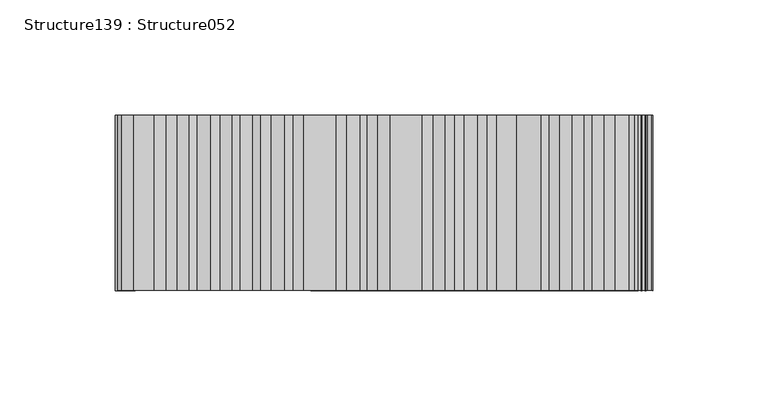
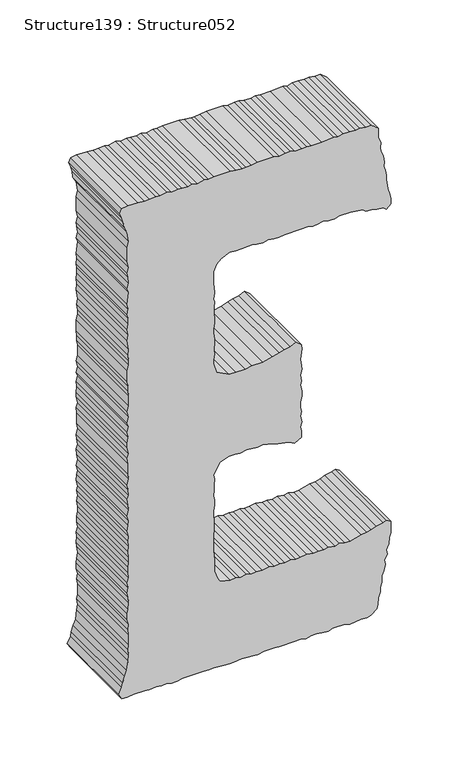
"""IFC4 building model written with IfcOpenShell, lengths in millimetres: proxy geometry, Structure139 : Structure052."""

from ifc_helpers import new_model, si_unit, frame, origin, place, context, project, spatial, polyline, outline, extrude, source, transform, mapped, element, save


def structure139_structure052_afdb430f(model_context):
    return source(origin(), model_context, "Body", "SweptSolid", [
        extrude(outline(polyline([(3552.242032, -42297.2179571), (3556.3417965, -42291.9580636), (3559.8671125, -42291.3563369), (3565.7094775, -42290.7770747), (3570.4109687, -42289.0152189), (3574.5107332, -42289.0152189), (3578.6104977, -42287.83423), (3584.4689087, -42287.83423), (3588.5702778, -42286.0964433), (3593.8285667, -42284.9154544), (3598.5284533, -42285.5171811), (3602.6298224, -42283.1552033), (3606.7295868, -42283.75693), (3611.4134274, -42281.9742144), (3617.2718384, -42281.3933476), (3620.7971545, -42280.2123587), (3625.472972, -42280.2123587), (3631.3410106, -42280.2123587), (3633.6821286, -42283.75693), (3632.5155811, -42286.6532411), (3631.3410106, -42292.5373258), (3629.5984101, -42296.6370903), (3628.4158166, -42300.7384594), (3627.8397636, -42305.4190907), (3625.472972, -42314.8012132), (3625.472972, -42319.4818445), (3626.6571701, -42324.1608712), (3625.472972, -42327.6829781), (3626.6571701, -42333.5429937), (3625.472972, -42337.6668272), (3626.0554434, -42342.3249941), (3625.472972, -42346.4247586), (3626.6571701, -42352.3088433), (3626.0554434, -42357.5687368), (3625.472972, -42361.6685013), (3626.6571701, -42365.7698704), (3625.472972, -42371.0506238), (3626.0554434, -42375.1519929), (3625.472972, -42379.8326242), (3626.6571701, -42384.5116509), (3625.472972, -42390.3957356), (3626.0554434, -42395.6556291), (3625.472972, -42400.3346558), (3626.6571701, -42403.8567627), (3625.472972, -42409.7183829), (3626.6571701, -42413.2388852), (3626.0554434, -42417.9195165), (3628.4158166, -42426.7223767), (3631.915459, -42429.0394256), (3638.9580681, -42431.4030081), (3648.9258713, -42431.4030081), (3654.1841602, -42431.9822703), (3657.7014533, -42432.5615325), (3671.7690209, -42432.5615325), (3677.0449605, -42431.9822703), (3685.8285655, -42431.9822703), (3689.3458585, -42432.5615325), (3694.029699, -42432.5615325), (3699.3136616, -42431.4030081), (3704.0135482, -42431.4030081), (3708.087639, -42432.5615325), (3712.2146818, -42431.9822703), (3716.8985223, -42431.9822703), (3722.7312597, -42431.4030081), (3726.2742264, -42432.5615325), (3733.8736333, -42428.4826279), (3736.2163558, -42426.7223767), (3739.1592005, -42419.1005054), (3739.1592005, -42413.7956829), (3738.5574738, -42409.7183829), (3739.7416719, -42403.8567627), (3739.1592005, -42400.3346558), (3738.5574738, -42394.4746402), (3739.1592005, -42390.3957356), (3737.400554, -42381.5928753), (3735.6146291, -42376.8897795), (3734.47536, -42371.0506238), (3733.2991849, -42366.9508593), (3730.9323932, -42362.8270257), (3734.47536, -42356.9894746), (3739.7416719, -42356.9894746), (3744.4158848, -42357.5687368), (3748.5429276, -42356.3877479), (3753.8012165, -42357.5687368), (3757.8753073, -42356.9894746), (3762.0023501, -42357.5687368), (3766.684586, -42357.5687368), (3771.3860772, -42356.3877479), (3776.6427615, -42356.3877479), (3781.9299333, -42357.5687368), (3785.4456218, -42356.9894746), (3791.3056374, -42357.5687368), (3795.960595, -42356.3877479), (3799.5051664, -42356.9894746), (3805.3459267, -42357.5687368), (3814.7296538, -42356.3877479), (3818.2309008, -42356.9894746), (3822.348316, -42361.6685013), (3820.015221, -42366.3715971), (3818.8310229, -42371.6314906), (3817.6741031, -42375.7312551), (3815.9154565, -42381.5928753), (3814.148787, -42389.7940089), (3814.148787, -42399.1536669), (3812.9726119, -42405.0377516), (3812.9726119, -42413.2388852), (3813.5743386, -42419.1005054), (3818.8310229, -42429.6186879), (3827.6162325, -42432.5615325), (3831.1575946, -42432.5615325), (3835.8334121, -42431.4030081), (3840.5172527, -42431.9822703), (3845.8012153, -42431.4030081), (3849.8753061, -42431.4030081), (3855.1769193, -42432.5615325), (3859.2606378, -42432.5615325), (3863.9332461, -42431.4030081), (3868.0618934, -42431.4030081), (3873.3185778, -42431.9822703), (3878.5784713, -42431.9822703), (3883.2863809, -42431.4030081), (3886.2051565, -42432.5615325), (3891.5067697, -42431.4030081), (3896.763454, -42431.9822703), (3900.2887701, -42432.5615325), (3910.8310217, -42432.5615325), (3916.6653636, -42429.6186879), (3920.7908018, -42426.1206501), (3923.7079727, -42418.4987787), (3923.1319197, -42413.2388852), (3923.7079727, -42408.537394), (3923.7079727, -42399.1536669), (3923.1319197, -42395.6556291), (3922.5494483, -42389.7940089), (3923.7079727, -42385.6926398), (3922.5494483, -42380.4118864), (3922.5494483, -42376.3105173), (3923.1319197, -42371.6314906), (3923.1319197, -42357.5687368), (3923.7079727, -42351.7071166), (3922.5494483, -42347.0040208), (3922.5494483, -42342.9267208), (3923.7079727, -42338.2460895), (3922.5494483, -42333.5429937), (3922.5494483, -42328.2847047), (3923.7079727, -42324.1608712), (3923.7079727, -42314.8012132), (3922.5494483, -42304.2381018), (3920.2067257, -42301.3177216), (3919.6066036, -42296.6370903), (3918.4480792, -42291.9580636), (3917.8479571, -42286.6532411), (3915.5068392, -42283.75693), (3919.6066036, -42280.2123587), (3924.2888396, -42280.2123587), (3928.4158823, -42280.8140853), (3933.6741713, -42282.5759411), (3937.1930689, -42283.1552033), (3942.4770315, -42283.75693), (3946.5511223, -42283.75693), (3951.2606365, -42284.9154544), (3955.360401, -42286.0964433), (3959.4617701, -42285.5171811), (3965.3201811, -42286.6532411), (3969.994394, -42288.4359567), (3973.5197101, -42289.0152189), (3977.6194746, -42288.4359567), (3983.4794902, -42290.7770747), (3988.1633307, -42290.7770747), (3991.6806238, -42290.7770747), (3996.390138, -42296.6370903), (3996.390138, -42301.3177216), (3996.9645864, -42306.6000796), (3996.390138, -42310.0981174), (3996.9645864, -42315.3804754), (3996.9645864, -42320.6628334), (3995.7803883, -42325.3418601), (3996.9645864, -42328.863967), (3995.7803883, -42339.4046139), (3995.7803883, -42348.1850097), (3996.390138, -42352.3088433), (3995.7803883, -42356.3877479), (3995.7803883, -42362.2477635), (3996.9645864, -42366.3715971), (3996.9645864, -42370.4488971), (3995.7803883, -42375.7312551), (3996.9645864, -42380.4118864), (3996.9645864, -42394.4746402), (3996.390138, -42399.7553936), (3995.7803883, -42404.4584894), (3995.7803883, -42407.3548005), (3996.390138, -42413.2388852), (3996.9645864, -42417.9195165), (3996.9645864, -42431.9822703), (3996.390138, -42436.661297), (3996.9645864, -42440.1834039), (3995.7803883, -42446.0450241), (3996.9645864, -42450.7465153), (3995.7803883, -42454.2461577), (3996.390138, -42459.5044466), (3996.390138, -42463.0265535), (3995.7803883, -42468.3089115), (3996.9645864, -42472.4086759), (3995.7803883, -42478.2702962), (3996.390138, -42481.768334), (3995.7803883, -42487.0731564), (3995.7803883, -42491.7537877), (3996.390138, -42497.0120767), (3996.390138, -42505.7940771), (3995.7803883, -42511.0972949), (3991.6806238, -42512.8366862), (3987.5792547, -42511.0972949), (3982.8793681, -42509.916306), (3977.6194746, -42509.3370438), (3972.3627903, -42506.3958038), (3964.1343784, -42505.2148149), (3958.8776941, -42506.3958038), (3945.9766739, -42506.3958038), (3940.718385, -42505.2148149), (3935.4328178, -42506.3958038), (3931.9058971, -42505.7940771), (3926.0490907, -42505.2148149), (3921.3748778, -42506.3958038), (3917.8479571, -42505.2148149), (3907.3313793, -42506.3958038), (3902.6314927, -42505.7940771), (3897.9476522, -42506.3958038), (3894.4030808, -42505.7940771), (3889.7208449, -42505.7940771), (3884.4609514, -42506.3958038), (3879.7610648, -42505.7940771), (3874.5043805, -42506.3958038), (3866.3032469, -42505.2148149), (3861.0192843, -42505.7940771), (3855.7353217, -42505.2148149), (3852.2340747, -42505.2148149), (3846.9757858, -42506.3958038), (3836.9919366, -42506.3958038), (3832.8921721, -42505.7940771), (3828.2163546, -42505.7940771), (3824.1149855, -42505.2148149), (3814.7296538, -42505.2148149), (3810.0474179, -42506.3958038), (3804.7730829, -42505.2148149), (3799.5051664, -42506.3958038), (3795.960595, -42505.2148149), (3791.3056374, -42506.3958038), (3786.6298199, -42505.7940771), (3781.3282066, -42506.3958038), (3777.2444882, -42506.3958038), (3771.3860772, -42505.2148149), (3767.8607611, -42506.3958038), (3762.5848215, -42505.7940771), (3753.2171405, -42505.7940771), (3748.5429276, -42505.2148149), (3743.2332913, -42506.3958038), (3739.1592005, -42505.7940771), (3733.8736333, -42505.2148149), (3730.3563402, -42506.3958038), (3725.0996559, -42505.7940771), (3720.4158154, -42505.2148149), (3715.1302482, -42506.3958038), (3710.4560353, -42505.2148149), (3706.9130685, -42505.7940771), (3701.6547796, -42506.3958038), (3696.3884676, -42505.2148149), (3692.2710525, -42505.7940771), (3687.587212, -42505.2148149), (3682.8857208, -42505.7940771), (3677.6274319, -42505.2148149), (3672.9435914, -42505.2148149), (3668.8261762, -42505.7940771), (3663.5598643, -42505.7940771), (3658.8840468, -42505.2148149), (3654.7842823, -42506.3958038), (3650.1004418, -42505.7940771), (3645.4262289, -42506.3958038), (3641.2991861, -42505.7940771), (3636.0408972, -42505.2148149), (3630.7392839, -42505.7940771), (3626.6571701, -42506.3958038), (3621.3732075, -42506.3958038), (3616.69739, -42505.2148149), (3612.0135494, -42505.7940771), (3607.3393366, -42505.2148149), (3597.9540049, -42505.2148149), (3593.8285667, -42505.7940771), (3588.5702778, -42505.2148149), (3583.8864372, -42505.7940771), (3575.6853037, -42506.975066), (3570.9854171, -42508.7353171), (3565.7094775, -42510.4955683), (3561.6257591, -42511.0972949), (3555.7416744, -42514.0176751), (3551.0658569, -42511.0972949), (3551.0658569, -42506.3958038), (3551.6675836, -42501.1134458), (3551.6675836, -42491.7537877), (3551.0658569, -42487.6524187), (3551.6675836, -42481.768334), (3551.0658569, -42477.0893073), (3551.6675836, -42473.0104026), (3550.4833855, -42468.3089115), (3550.4833855, -42463.6282801), (3551.6675836, -42458.9251844), (3551.6675836, -42440.7626661), (3551.0658569, -42436.0820348), (3551.6675836, -42431.9822703), (3550.4833855, -42421.4175543), (3550.4833855, -42417.3402543), (3551.0658569, -42412.0578963), (3551.6675836, -42408.537394), (3551.0658569, -42403.2775005), (3551.0658569, -42398.5968691), (3550.4833855, -42394.4746402), (3551.6675836, -42389.2147467), (3551.6675836, -42379.8326242), (3551.0658569, -42376.3105173), (3551.0658569, -42362.2477635), (3551.6675836, -42357.5687368), (3550.4833855, -42352.8881055), (3551.6675836, -42348.7867364), (3551.6675836, -42344.1077097), (3551.0658569, -42339.4046139), (3550.4833855, -42333.5429937), (3551.6675836, -42330.0449559), (3551.6675836, -42319.4818445), (3550.4833855, -42315.3804754), (3551.6675836, -42306.0208174), (3551.0658569, -42300.7384594), (3552.242032, -42297.2179571)])), frame((0.0, 247945.1599557, 0.0), z_axis=(0.0, 1.0, 0.0), x_axis=(0.0, 0.0, 1.0)), (0.0, 0.0, 1.0), 76.2),
    ])


if __name__ == "__main__":
    model = new_model("IFC4")
    model_context = context("Model", 3, world=origin())
    ifc_project = project(units=[si_unit("LENGTHUNIT", "METRE", prefix="MILLI")], contexts=[model_context])
    site = spatial("IfcSite", under=ifc_project)
    building = spatial("IfcBuilding", under=site)
    placement = place(None, origin())
    structure139_structure052_shape = structure139_structure052_afdb430f(model_context)
    element("IfcBuildingElementProxy", 1, Name="Structure139 : Structure052", ObjectType="Structure139 : Structure052", at=placement, inside=building, context=model_context, shape_type="MappedRepresentation", body=[
        mapped(structure139_structure052_shape, transform((0.0, 0.0, 0.0), x_axis=(1.0, 0.0, 0.0), y_axis=(0.0, 1.0, 0.0), z_axis=(0.0, 0.0, 1.0))),
    ])
    save(model, "model.ifc")

# Revit data of these elements
# Type "Structure139 : Structure052"
#   NameOverride = "Structure052"
# Element 1 (IfcBuildingElementProxy, "Structure139 : Structure052")
#   Materials on its faces: "BRUSHED ALUM. LETTERING"
# Materials
#   "BRUSHED ALUM. LETTERING": class "Unassigned", colour RGB 169 181 186, transparency 0, Cost = 0
